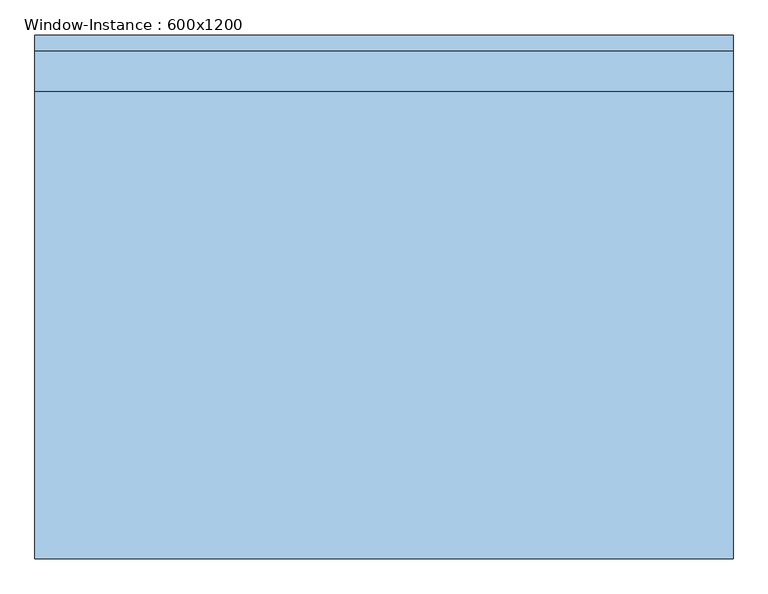
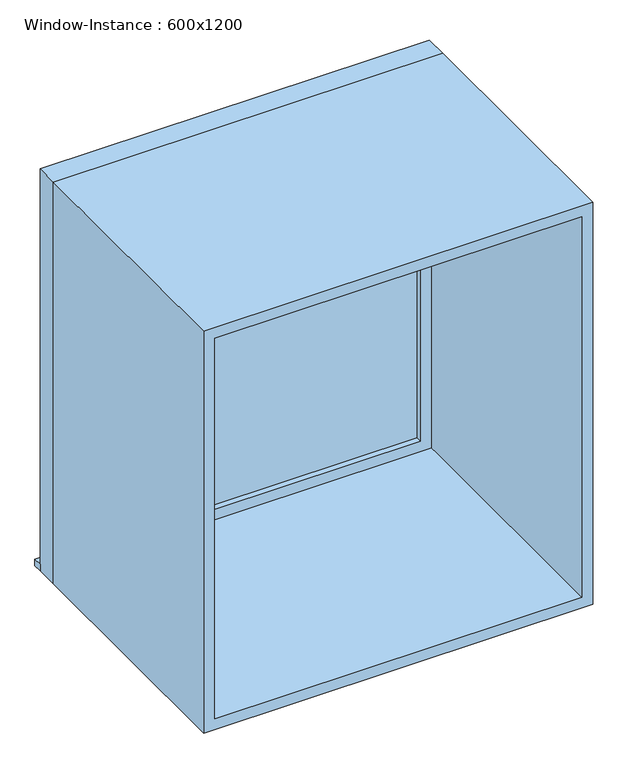
"""IFC4 building model written with IfcOpenShell, lengths in millimetres: window geometry, Window-Instance : 600x1200."""

from ifc_helpers import new_model, si_unit, frame, origin, place, context, project, spatial, polyline, outline, extrude, source, transform, mapped, element, save


def window_instance_600x1200_c71d64f5(model_context):
    return source(origin(), model_context, "Body", "SweptSolid", [
        extrude(outline(polyline([(-588.1, 425.4), (511.9, 425.4), (511.9, 400.0), (-588.1, 400.0), (-588.1, 425.4)])), frame((0.0, 0.0, 900.0), z_axis=(0.0, 0.0, 1.0), x_axis=(1.0, 0.0, 0.0)), (0.0, 0.0, 1.0), 19.05),
        extrude(outline(polyline([(448.4, 351.425), (-524.6, 351.425), (-524.6, 364.125), (448.4, 364.125), (448.4, 351.425)])), frame((0.0, 0.0, 963.5), z_axis=(0.0, 0.0, 1.0), x_axis=(1.0, 0.0, 0.0)), (0.0, 0.0, 1.0), 1073.0),
        extrude(outline(polyline([(2080.95, -569.05), (919.05, -569.05), (919.05, 492.85), (2080.95, 492.85), (2080.95, -569.05)]), holes=[polyline([(2036.5, -524.6), (2036.5, 448.4), (963.5, 448.4), (963.5, -524.6), (2036.5, -524.6)])]), frame((0.0, 335.55, 0.0), z_axis=(0.0, 1.0, 0.0), x_axis=(0.0, 0.0, 1.0)), (0.0, 0.0, 1.0), 44.45),
        extrude(outline(polyline([(2100.0, -588.1), (900.0, -588.1), (900.0, 511.9), (2100.0, 511.9), (2100.0, -588.1)]), holes=[polyline([(2068.25, -556.35), (2068.25, 480.15), (931.75, 480.15), (931.75, -556.35), (2068.25, -556.35)])]), frame((0.0, -400.0, 0.0), z_axis=(0.0, 1.0, 0.0), x_axis=(0.0, 0.0, 1.0)), (0.0, 0.0, 1.0), 735.55),
        extrude(outline(polyline([(2100.0, 511.9), (2100.0, -588.1), (900.0, -588.1), (900.0, 511.9), (2100.0, 511.9)]), holes=[polyline([(2080.95, 492.85), (919.05, 492.85), (919.05, -569.05), (2080.95, -569.05), (2080.95, 492.85)])]), frame((0.0, 335.55, 0.0), z_axis=(0.0, 1.0, 0.0), x_axis=(0.0, 0.0, 1.0)), (0.0, 0.0, 1.0), 64.45),
    ])


if __name__ == "__main__":
    model = new_model("IFC4")
    model_context = context("Model", 3, world=origin())
    ifc_project = project(units=[si_unit("LENGTHUNIT", "METRE", prefix="MILLI")], contexts=[model_context])
    site = spatial("IfcSite", under=ifc_project)
    building = spatial("IfcBuilding", under=site)
    placement = place(None, origin())
    window_instance_600x1200_shape = window_instance_600x1200_c71d64f5(model_context)
    element("IfcWindow", 1, ObjectType="Window-Instance : 600x1200", at=placement, inside=building, context=model_context, shape_type="MappedRepresentation", body=[
        mapped(window_instance_600x1200_shape, transform((0.0, 0.0, 0.0), x_axis=(1.0, 0.0, 0.0), y_axis=(0.0, 1.0, 0.0), z_axis=(0.0, 0.0, 1.0))),
    ])
    save(model, "model.ifc")

# Revit data of these elements
# Type "Window-Instance : 600x1200"
#   Type Mark = "7"
#   Construction Type Id = "GSP4R"
#   Assembly Code = "B2020100"
#   Analytic Construction = "1/8 in Pilkington single glazing"
#   Visual Light Transmittance = 0.9
#   Thermal Resistance (R) = 0.149095 (m²·K)/W
#   Solar Heat Gain Coefficient = 0.86
#   Heat Transfer Coefficient (U) = 6.70716 W/(m²·K)
#   Height [instance default] = 1200 mm
#   Default Sill Height = 900 mm
#   Width [instance default] = 600 mm
#   Window Inset = 20 mm
#   Glass Pane Material = WW-EC-GL-Storefront
#   Sash Material = WW-EC-RGB-White
#   Wall Closure = (empty or 0)
# Element 1 (IfcWindow, "Window-Instance : 600x1200")
#   Width = 1100 mm
#   Materials on its faces: "WW-EC-RGB-White", "WW-EC-GL-Storefront"
# Materials
#   "WW-EC-GL-Storefront": class "Glass", colour RGB 236 240 239, transparency 0.85, Description = "Storefront Glass", Cost = 0
#   "WW-EC-RGB-White": class "Generic", colour RGB 255 255 255, transparency 0, Comments = "If region requests off-white, swith asset color to RGB 231-228-220", Description = "Generic Color", Cost = 0
